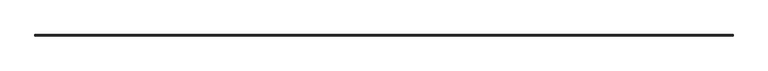
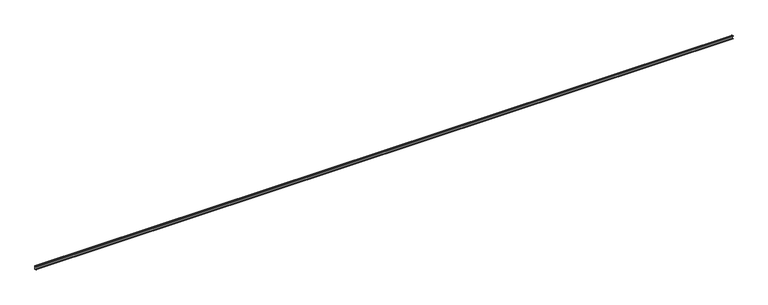
"""IFC4 building model written with IfcOpenShell, lengths in millimetres: beam geometry, 0912_Steel Framing_LC_KDS3530 : H_SB_AR_B03_LC-200x75x25x3.2."""

from ifc_helpers import new_model, si_unit, point, frame, frame_2d, origin, place, context, project, spatial, polyline, circle_curve, trimmed, segment, composite_curve, outline, extrude, source, transform, mapped, element, save


def beam_1c327814(model_context):
    return source(origin(), model_context, "Body", "SweptSolid", [
        extrude(outline(composite_curve([segment(polyline([(18.6, 87.5), (18.6, -87.5)]), True, "CONTINUOUS"), segment(trimmed(circle_curve(frame_2d((6.1, -87.5)), 12.5), [point((18.6, -87.5))], [point((6.1, -100.0))], False, "CARTESIAN"), True, "CONTINUOUS"), segment(polyline([(6.1, -100.0), (-43.9, -100.0)]), True, "CONTINUOUS"), segment(trimmed(circle_curve(frame_2d((-43.9, -87.5)), 12.5), [point((-43.9, -100.0))], [point((-56.4, -87.5))], False, "CARTESIAN"), True, "CONTINUOUS"), segment(polyline([(-56.4, -87.5), (-56.4, -75.0), (-51.9, -75.0), (-51.9, -87.5)]), True, "CONTINUOUS"), segment(trimmed(circle_curve(frame_2d((-43.9, -87.5)), 8.0), [point((-51.9, -87.5))], [point((-43.9, -95.5))], True, "CARTESIAN"), True, "CONTINUOUS"), segment(polyline([(-43.9, -95.5), (6.1, -95.5)]), True, "CONTINUOUS"), segment(trimmed(circle_curve(frame_2d((6.1, -87.5)), 8.0), [point((6.1, -95.5))], [point((14.1, -87.5))], True, "CARTESIAN"), True, "CONTINUOUS"), segment(polyline([(14.1, -87.5), (14.1, 87.5)]), True, "CONTINUOUS"), segment(trimmed(circle_curve(frame_2d((6.1, 87.5)), 8.0), [point((14.1, 87.5))], [point((6.1, 95.5))], True, "CARTESIAN"), True, "CONTINUOUS"), segment(polyline([(6.1, 95.5), (-41.1, 95.5)]), True, "CONTINUOUS"), segment(trimmed(circle_curve(frame_2d((-41.1, 87.5)), 8.0), [point((-41.1, 95.5))], [point((-49.1, 87.5))], True, "CARTESIAN"), True, "CONTINUOUS"), segment(polyline([(-49.1, 87.5), (-49.1, 75.0), (-53.6, 75.0), (-53.6, 87.5)]), True, "CONTINUOUS"), segment(trimmed(circle_curve(frame_2d((-41.1, 87.5)), 12.5), [point((-53.6, 87.5))], [point((-41.1, 100.0))], False, "CARTESIAN"), True, "CONTINUOUS"), segment(polyline([(-41.1, 100.0), (6.1, 100.0)]), True, "CONTINUOUS"), segment(trimmed(circle_curve(frame_2d((6.1, 87.5)), 12.5), [point((6.1, 100.0))], [point((18.6, 87.5))], False, "CARTESIAN"), True, "CONTINUOUS")], self_intersect=False)), frame((-19725.0, 0.0, 0.0), z_axis=(1.0, 0.0, 0.0), x_axis=(0.0, 1.0, 0.0)), (0.0, 0.0, 1.0), 39450.0),
    ])


if __name__ == "__main__":
    model = new_model("IFC4")
    model_context = context("Model", 3, world=origin())
    ifc_project = project(units=[si_unit("LENGTHUNIT", "METRE", prefix="MILLI")], contexts=[model_context])
    site = spatial("IfcSite", under=ifc_project)
    building = spatial("IfcBuilding", under=site)
    placement = place(None, origin())
    beam_shape = beam_1c327814(model_context)
    element("IfcBeam", 1, ObjectType="0912_Steel Framing_LC_KDS3530 : H_SB_AR_B03_LC-200x75x25x3.2", at=placement, inside=building, context=model_context, shape_type="MappedRepresentation", body=[
        mapped(beam_shape, transform((0.0, 0.0, 0.0), x_axis=(1.0, 0.0, 0.0), y_axis=(0.0, 1.0, 0.0), z_axis=(0.0, 0.0, 1.0))),
    ])
    save(model, "model.ifc")

# Revit data of these elements
# Type "0912_Steel Framing_LC_KDS3530 : H_SB_AR_B03_LC-200x75x25x3.2"
#   r = 8 mm
#   d = 25 mm
#   R = 11.2 mm
#   Perimeter = 0.78 m²/m
#   Nominal Weight = 14.00 kgf/m
#   Length [instance default] = 1000 mm
#   B = 75 mm
#   H = 200 mm
#   tw = 3.2 mm
#   x = 18.6 mm
#   A = 1.00 m²
#   Structural Material [instance default] = Steel, 45-345
#   Assembly Code = ""
# Element 1 (IfcBeam, "0912_Steel Framing_LC_KDS3530 : H_SB_AR_B03_LC-200x75x25x3.2")
#   Structural Material = Steel ASTM A36
#   Materials on its faces: "Steel ASTM A36"
# Materials
#   "Steel, 45-345": class "Metal", colour RGB 189 187 185, transparency 0, Description = "Steel 345 MPa", Cost = 0
#   "Steel ASTM A36": class "Metal", colour RGB 199 199 199, transparency 0, Description = "Structural steel, ASTM A36 Grade B, mill finish", Cost = 0
